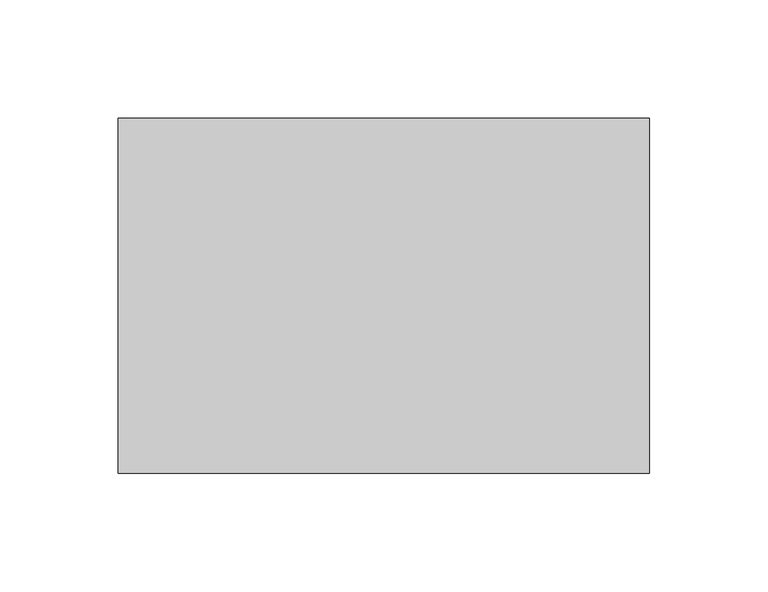
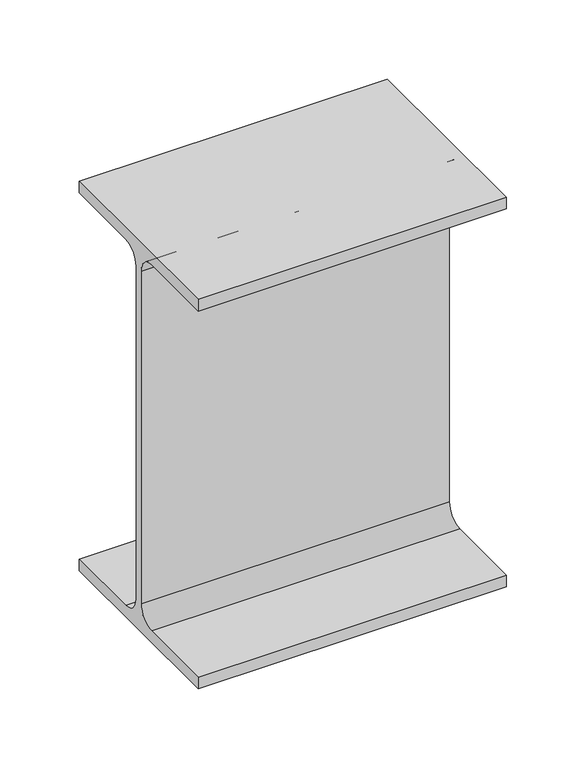
"""IFC4 building model written with IfcOpenShell, lengths in millimetres: beam geometry, 0912_Steel Framing_H-KSD3502 : H_SB_ASB_H-300x150x6.5x9."""

from ifc_helpers import new_model, si_unit, point, frame, frame_2d, origin, place, context, project, spatial, polyline, circle_curve, trimmed, segment, composite_curve, outline, extrude, source, transform, mapped, element, save


def beam_8d7e8f50(model_context):
    return source(origin(), model_context, "Body", "SweptSolid", [
        extrude(outline(composite_curve([segment(polyline([(75.0, -141.0), (75.0, -150.0), (-75.0, -150.0), (-75.0, -141.0), (-16.25, -141.0)]), True, "CONTINUOUS"), segment(trimmed(circle_curve(frame_2d((-16.25, -128.0)), 13.0), [point((-16.25, -141.0))], [point((-3.25, -128.0))], True, "CARTESIAN"), True, "CONTINUOUS"), segment(polyline([(-3.25, -128.0), (-3.25, 128.0)]), True, "CONTINUOUS"), segment(trimmed(circle_curve(frame_2d((-16.25, 128.0)), 13.0), [point((-3.25, 128.0))], [point((-16.25, 141.0))], True, "CARTESIAN"), True, "CONTINUOUS"), segment(polyline([(-16.25, 141.0), (-75.0, 141.0), (-75.0, 150.0), (75.0, 150.0), (75.0, 141.0), (16.25, 141.0)]), True, "CONTINUOUS"), segment(trimmed(circle_curve(frame_2d((16.25, 128.0)), 13.0), [point((16.25, 141.0))], [point((3.25, 128.0))], True, "CARTESIAN"), True, "CONTINUOUS"), segment(polyline([(3.25, 128.0), (3.25, -128.0)]), True, "CONTINUOUS"), segment(trimmed(circle_curve(frame_2d((16.25, -128.0)), 13.0), [point((3.25, -128.0))], [point((16.25, -141.0))], True, "CARTESIAN"), True, "CONTINUOUS"), segment(polyline([(16.25, -141.0), (75.0, -141.0)]), True, "CONTINUOUS")], self_intersect=False)), frame((-37.3, 0.0, 0.0), z_axis=(1.0, 0.0, 0.0), x_axis=(0.0, 1.0, 0.0)), (0.0, 0.0, 1.0), 224.5999994),
    ])


if __name__ == "__main__":
    model = new_model("IFC4")
    model_context = context("Model", 3, world=origin())
    ifc_project = project(units=[si_unit("LENGTHUNIT", "METRE", prefix="MILLI")], contexts=[model_context])
    site = spatial("IfcSite", under=ifc_project)
    building = spatial("IfcBuilding", under=site)
    placement = place(None, origin())
    beam_shape = beam_8d7e8f50(model_context)
    element("IfcBeam", 1, ObjectType="0912_Steel Framing_H-KSD3502 : H_SB_ASB_H-300x150x6.5x9", at=placement, inside=building, context=model_context, shape_type="MappedRepresentation", body=[
        mapped(beam_shape, transform((0.0, 0.0, 0.0), x_axis=(1.0, 0.0, 0.0), y_axis=(0.0, 1.0, 0.0), z_axis=(0.0, 0.0, 1.0))),
    ])
    save(model, "model.ifc")

# Revit data of these elements
# Type "0912_Steel Framing_H-KSD3502 : H_SB_ASB_H-300x150x6.5x9"
#   H_WM Code_1 = "S01AA002-00001 | Main Steel Structure Fabrication Work | Shelter/Building | Medium Steel - Standard (90KG/M>Weight≥30KG/M) | Material: (   )"
#   H_WM Code_2 = "S03AA028-00001 | Main Steel Structure Erection Work | Shelter/Building | Medium Steel (90KG/M>Weight≥30KG/M) | Material: (   )"
#   H_WM Code_3 = "S01AA010-00001 | Main Steel Structure Fabrication Work | Shelter/Building | Steel Painting/Coating | for Non-Fireproofed Steel Surface, Surface Preparation, Primer, Second & Final Coat | Material: (   )"
#   H_Q'ty Cal Type Tag = "SB-Q2"
#   Width = 15.0 cm
#   Web Thickness = 0.65 cm
#   Web Fillet = 1.3 cm
#   Warping Constant = 107000.0 cm⁶
#   W = 0
#   Torsional Moment of Inertia = 9.9539 cm⁴
#   Section Area = 46.78 cm²
#   Plastic Modulus weak axis = 105.0 cm³
#   Plastic Modulus strong axis = 542.0 cm³
#   Perimeter = 1.17 m²/m
#   Nominal Weight = 36.70 kgf/m
#   Moment of Inertia weak axis = 508.00 cm⁴
#   Moment of Inertia strong axis = 7210.00 cm⁴
#   Height = 30.0 cm
#   Flange Thickness = 0.9 cm
#   Elastic Modulus weak axis = 67.7 cm³
#   Elastic Modulus strong axis = 481.0 cm³
#   Centroid Vertical = 15.0 cm
#   Centroid Horizontal = 7.5 cm
#   Ix = 72100000
#   Length [instance default] = 1.5240 m
#   Zx = 542000
#   b = 0.1500 m
#   h = 0.3000 m
#   r = 0.0130 m
#   s = 0.0065 m
#   t = 0.0090 m
#   A = 0.004678 m²
#   Structural Material [instance default] = Steel, 45-345
#   Assembly Code = ""
# Element 1 (IfcBeam, "0912_Steel Framing_H-KSD3502 : H_SB_ASB_H-300x150x6.5x9")
#   Structural Material = none
# Materials
#   "Steel, 45-345": class "Metal", colour RGB 189 187 185, transparency 0, Description = "Steel 345 MPa", Cost = 0
